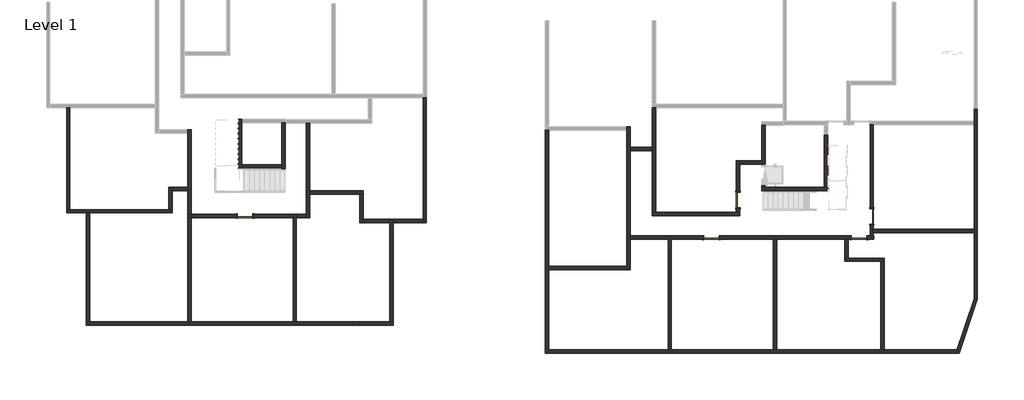
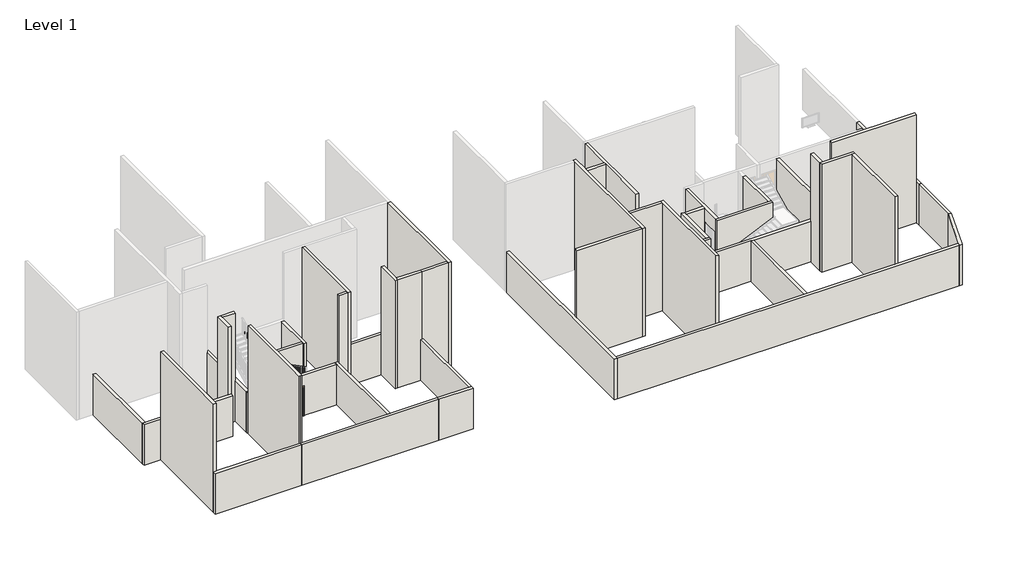
# One storey, part 1 of 3: 47 walls, 5 doors.
# Revit data of these elements (continued)
# Area at (20066.111, 5871.007) mm, upper offset 243.84 cm, lower offset 0 cm
#   Number = "12"
#   Name = "Area"
# Room, not placed, phase "New Construction", upper offset 0 cm, lower offset 0 cm
#   Number = "57"
#   Name = "Room"
# Room, not placed, phase "New Construction", upper offset 0 cm, lower offset 0 cm
#   Number = ""
#   Name = "Room"
# Room, not placed, phase "New Construction", upper offset 0 cm, lower offset 0 cm
#   Number = "59"
#   Name = "Room"
# Room, not placed, phase "New Construction", upper offset 0 cm, lower offset 0 cm
#   Number = "60"
#   Name = "Room"
# Room, not placed, phase "New Construction", upper offset 0 cm, lower offset 0 cm
#   Number = "61"
#   Name = "Room"
# Room, not placed, phase "New Construction", upper offset 0 cm, lower offset 0 cm
#   Number = "62"
#   Name = "Room"
# Room, not placed, phase "New Construction", upper offset 0 cm, lower offset 0 cm
#   Number = "63"
#   Name = "Room"
# Area, not placed, upper offset 0 cm, lower offset 0 cm
#   Number = "5"
#   Name = "Dere Parsel Toplam Alan"
# Room, not placed, phase "New Construction", upper offset 0 cm, lower offset 0 cm
#   Number = "67"
#   Name = "Room"
# Room, not placed, phase "New Construction", upper offset 0 cm, lower offset 0 cm
#   Number = "68"
#   Name = "Room"
# Room at (-14817.024, 11588.139) mm, phase "New Construction", upper level "Level 1", upper offset 243.84 cm, lower offset 0 cm
#   Number = "139"
#   Name = "Room"
# Room at (27717.749, -8269.379) mm, phase "New Construction", upper level "Level 1", upper offset 243.84 cm, lower offset 0 cm
#   Number = "90"
#   Name = "3"
# Area, not placed, upper offset 0 cm, lower offset 0 cm
#   Number = "6"
#   Name = "Area"
# Room, not placed, phase "New Construction", upper offset 0 cm, lower offset 0 cm
#   Number = "93"
#   Name = "6"
# Room, not placed, phase "New Construction", upper offset 0 cm, lower offset 0 cm
#   Number = "5"
#   Name = "Room"
# Room, not placed, phase "New Construction", upper offset 0 cm, lower offset 0 cm
#   Number = "6"
#   Name = "Room"
# Room, not placed, phase "New Construction", upper offset 0 cm, lower offset 0 cm
#   Number = "124"
#   Name = "Room"
# Room at (-20992.701, 5104.389) mm, phase "New Construction", upper level "Level 1", upper offset 243.84 cm, lower offset 0 cm
#   Number = "140"
#   Name = "Room"
# Room at (-18388.177, -2994.154) mm, phase "New Construction", upper level "Level 1", upper offset 243.84 cm, lower offset 0 cm
#   Number = "141"
#   Name = "Room"
# Room, not placed, phase "New Construction", upper offset 0 cm, lower offset 0 cm
#   Number = "34"
#   Name = "Room"
# Room, not placed, phase "New Construction", upper offset 0 cm, lower offset 0 cm
#   Number = "35"
#   Name = "Room"
# Room, not placed, phase "New Construction", upper offset 0 cm, lower offset 0 cm
#   Number = "9"
#   Name = "Room"
# Room, not placed, phase "New Construction", upper offset 0 cm, lower offset 0 cm
#   Number = "10"
#   Name = "Room"
# Room, not placed, phase "New Construction", upper offset 0 cm, lower offset 0 cm
#   Number = "125"
#   Name = "Room"
# Room, not placed, phase "New Construction", upper offset 0 cm, lower offset 0 cm
#   Number = "126"
#   Name = "Room"
# Room, not placed, phase "New Construction", upper offset 0 cm, lower offset 0 cm
#   Number = "127"
#   Name = "Room"
# Room, not placed, phase "New Construction", upper offset 0 cm, lower offset 0 cm
#   Number = "128"
#   Name = "Room"
# Room, not placed, phase "New Construction", upper offset 0 cm, lower offset 0 cm
#   Number = "129"
#   Name = "Room"
# Room, not placed, phase "New Construction", upper offset 0 cm, lower offset 0 cm
#   Number = "91"
#   Name = "Room"
# Room at (-21021.225, 8802.195) mm, phase "New Construction", upper level "Level 1", upper offset 243.84 cm, lower offset 0 cm
#   Number = "130"
#   Name = "Room"
# Room at (-7278.952, -9510.79) mm, phase "New Construction", upper level "Level 1", upper offset 243.84 cm, lower offset 0 cm
#   Number = "131"
#   Name = "Room"
# Room, not placed, phase "New Construction", upper offset 0 cm, lower offset 0 cm
#   Number = "132"
#   Name = "Room"
# Room, not placed, phase "New Construction", upper offset 0 cm, lower offset 0 cm
#   Number = "133"
#   Name = "Room"
# Room, not placed, phase "New Construction", upper offset 0 cm, lower offset 0 cm
#   Number = ""
#   Name = ""
# Room, not placed, phase "New Construction", upper offset 0 cm, lower offset 0 cm
#   Number = "70"
#   Name = "Room"
# Room, not placed, phase "New Construction", upper offset 0 cm, lower offset 0 cm
#   Number = "71"
#   Name = "Room"
# Room, not placed, phase "New Construction", upper offset 0 cm, lower offset 0 cm
#   Number = "92"
#   Name = "Room"
# Room, not placed, phase "New Construction", upper offset 0 cm, lower offset 0 cm
#   Number = ""
#   Name = ""
# Area, not placed, upper offset 0 cm, lower offset 0 cm
#   Number = "10"
#   Name = "Area"
# Area, not placed, upper offset 0 cm, lower offset 0 cm
#   Number = "11"
#   Name = "Area"
# Room, not placed, phase "New Construction", upper offset 0 cm, lower offset 0 cm
#   Number = ""
#   Name = ""
# Room, not placed, phase "New Construction", upper offset 0 cm, lower offset 0 cm
#   Number = "37"
#   Name = "Room"
# Room, not placed, phase "New Construction", upper offset 0 cm, lower offset 0 cm
#   Number = ""
#   Name = "Banyo"
# Room, not placed, phase "New Construction", upper offset 0 cm, lower offset 0 cm
#   Number = ""
#   Name = ""
# Room, not placed, phase "New Construction", upper offset 0 cm, lower offset 0 cm
#   Number = ""
#   Name = "Yatak Odası"
# Room, not placed, phase "New Construction", upper offset 0 cm, lower offset 0 cm
#   Number = "39"
#   Name = "Room"
# Room, not placed, phase "New Construction", upper offset 0 cm, lower offset 0 cm
#   Number = ""
#   Name = "Salon-Mutfak"
# Area, not placed, upper offset 0 cm, lower offset 0 cm
#   Number = "9"
#   Name = "Area"
# Room, not placed, phase "New Construction", upper offset 0 cm, lower offset 0 cm
#   Number = "134"
#   Name = "Room"
# Room, not placed, phase "New Construction", upper offset 0 cm, lower offset 0 cm
#   Number = "135"
#   Name = "Room"
# Room, not placed, phase "New Construction", upper offset 0 cm, lower offset 0 cm
#   Number = "40"
#   Name = "Room"
# Room, not placed, phase "New Construction", upper offset 0 cm, lower offset 0 cm
#   Number = "41"
#   Name = "Room"
# Room at (-12898.035, -7311.307) mm, phase "New Construction", upper level "Level 1", upper offset 243.84 cm, lower offset 0 cm
#   Number = "142"
#   Name = "Room"
# Room, not placed, phase "New Construction", upper offset 0 cm, lower offset 0 cm
#   Number = "143"
#   Name = "Room"
# Room, not placed, phase "New Construction", upper offset 0 cm, lower offset 0 cm
#   Number = "144"
#   Name = "Room"
# Room at (-12608.918, 6284.855) mm, phase "New Construction", upper level "Level 1", upper offset 243.84 cm, lower offset 0 cm
#   Number = "145"
#   Name = "Room"
# Room at (-4085.235, 4670.303) mm, phase "New Construction", upper level "Level 1", upper offset 243.84 cm, lower offset 0 cm
#   Number = "146"
#   Name = "Room"
# Area, not placed, upper offset 0 cm, lower offset 0 cm
#   Number = "8"
#   Name = "Dere Parsel Toplam Alan"
# Room, not placed, phase "New Construction", upper offset 0 cm, lower offset 0 cm
#   Number = "108"
#   Name = "ASANSÖR"
# Room, not placed, phase "New Construction", upper offset 0 cm, lower offset 0 cm
#   Number = "89"
#   Name = "Room"
# Room at (-3408.462, -2181.87) mm, phase "New Construction", upper level "Level 1", upper offset 243.84 cm, lower offset 0 cm
#   Number = "147"
#   Name = "Room"
# Room, not placed, phase "New Construction", upper offset 0 cm, lower offset 0 cm
#   Number = "19"
#   Name = "Room"
# Room, not placed, phase "New Construction", upper offset 0 cm, lower offset 0 cm
#   Number = ""
#   Name = ""
# Room, not placed, phase "New Construction", upper offset 0 cm, lower offset 0 cm
#   Number = "21"
#   Name = "Room"
# Room, not placed, phase "New Construction", upper offset 0 cm, lower offset 0 cm
#   Number = "22"
#   Name = "Room"
# Room, not placed, phase "New Construction", upper offset 0 cm, lower offset 0 cm
#   Number = "23"
#   Name = "Room"
# Room, not placed, phase "New Construction", upper offset 0 cm, lower offset 0 cm
#   Number = "24"
#   Name = "Room"
# Room, not placed, phase "New Construction", upper offset 0 cm, lower offset 0 cm
#   Number = "25"
#   Name = "Room"
# Room, not placed, phase "New Construction", upper offset 0 cm, lower offset 0 cm
#   Number = "64"
#   Name = "Room"
# Room, not placed, phase "New Construction", upper offset 0 cm, lower offset 0 cm
#   Number = "65"
#   Name = "Room"
# Room, not placed, phase "New Construction", upper offset 0 cm, lower offset 0 cm
#   Number = "66"
#   Name = "Room"
# Room, not placed, phase "New Construction", upper offset 0 cm, lower offset 0 cm
#   Number = ""
#   Name = ""
# Room, not placed, phase "New Construction", upper offset 0 cm, lower offset 0 cm
#   Number = "27"
#   Name = "Room"
# Room, not placed, phase "New Construction", upper offset 0 cm, lower offset 0 cm
#   Number = "42"
#   Name = "Room"
# Area, not placed, upper offset 0 cm, lower offset 0 cm
#   Number = "13"
#   Name = "Area"
# Area at (-14699.602, 13833.859) mm, upper offset 243.84 cm, lower offset 0 cm
#   Number = "14"
#   Name = "Area"
# Area, not placed, upper offset 0 cm, lower offset 0 cm
#   Number = "2"
#   Name = "Area"
# Room, not placed, phase "New Construction", upper offset 0 cm, lower offset 0 cm
#   Number = "43"
#   Name = "Room"
# Room, not placed, phase "New Construction", upper offset 0 cm, lower offset 0 cm
#   Number = ""
#   Name = ""
# Room, not placed, phase "New Construction", upper offset 0 cm, lower offset 0 cm
#   Number = "94"
#   Name = "Room"
# Room, not placed, phase "New Construction", upper offset 0 cm, lower offset 0 cm
#   Number = ""
#   Name = ""
# Room, not placed, phase "New Construction", upper offset 0 cm, lower offset 0 cm
#   Number = "136"
#   Name = "Room"
# Room, not placed, phase "New Construction", upper offset 0 cm, lower offset 0 cm
#   Number = "1"
#   Name = "Room"
# Area, not placed, upper offset 0 cm, lower offset 0 cm
#   Number = "3"
#   Name = "Area"
# Room, not placed, phase "New Construction", upper offset 0 cm, lower offset 0 cm
#   Number = "7"
#   Name = "Room"
# Room, not placed, phase "New Construction", upper offset 0 cm, lower offset 0 cm
#   Number = "8"
#   Name = "Room"
# Room, not placed, phase "New Construction", upper offset 0 cm, lower offset 0 cm
#   Number = "2"
#   Name = "Room"
# Room, not placed, phase "New Construction", upper offset 0 cm, lower offset 0 cm
#   Number = "46"
#   Name = "Room"
# Room, not placed, phase "New Construction", upper offset 0 cm, lower offset 0 cm
#   Number = "3"
#   Name = "Room"
# Room, not placed, phase "New Construction", upper offset 0 cm, lower offset 0 cm
#   Number = ""
#   Name = ""
# Room, not placed, phase "New Construction", upper offset 0 cm, lower offset 0 cm
#   Number = "4"
#   Name = "Room"
# Area, not placed, upper offset 0 cm, lower offset 0 cm
#   Number = "1"
#   Name = "Area"
# Room, not placed, phase "New Construction", upper offset 0 cm, lower offset 0 cm
#   Number = ""
#   Name = ""
# Room, not placed, phase "New Construction", upper offset 0 cm, lower offset 0 cm
#   Number = "29"
#   Name = "Room"
# Area, not placed, upper offset 0 cm, lower offset 0 cm
#   Number = "7"
#   Name = "Dere Parsel Toplam Alan"
# Room, not placed, phase "New Construction", upper offset 0 cm, lower offset 0 cm
#   Number = "95"
#   Name = "ASANSÖR"
# Room, not placed, phase "New Construction", upper offset 0 cm, lower offset 0 cm
#   Number = "96"
#   Name = "Room"
# Room, not placed, phase "New Construction", upper offset 0 cm, lower offset 0 cm
#   Number = "97"
#   Name = "7"
# Room, not placed, phase "New Construction", upper offset 0 cm, lower offset 0 cm
#   Number = "98"
#   Name = "8"
# Room, not placed, phase "New Construction", upper offset 0 cm, lower offset 0 cm
#   Number = "99"
#   Name = "9"
# Room, not placed, phase "New Construction", upper offset 0 cm, lower offset 0 cm
#   Number = "100"
#   Name = "1"
# Room, not placed, phase "New Construction", upper offset 0 cm, lower offset 0 cm
#   Number = "101"
#   Name = "5"
# Room, not placed, phase "New Construction", upper offset 0 cm, lower offset 0 cm
#   Number = "102"
#   Name = "2"
# Room, not placed, phase "New Construction", upper offset 0 cm, lower offset 0 cm
#   Number = "103"
#   Name = "4"
# Room, not placed, phase "New Construction", upper offset 0 cm, lower offset 0 cm
#   Number = "104"
#   Name = "3"
# Room, not placed, phase "New Construction", upper offset 0 cm, lower offset 0 cm
#   Number = "105"
#   Name = "6"
